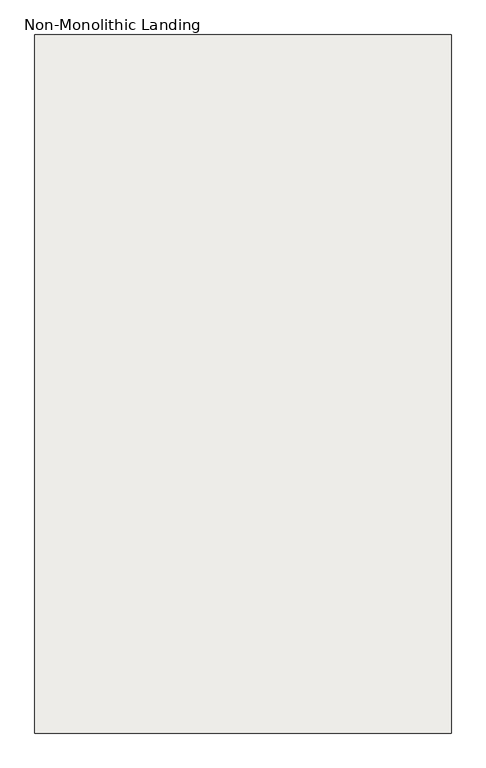
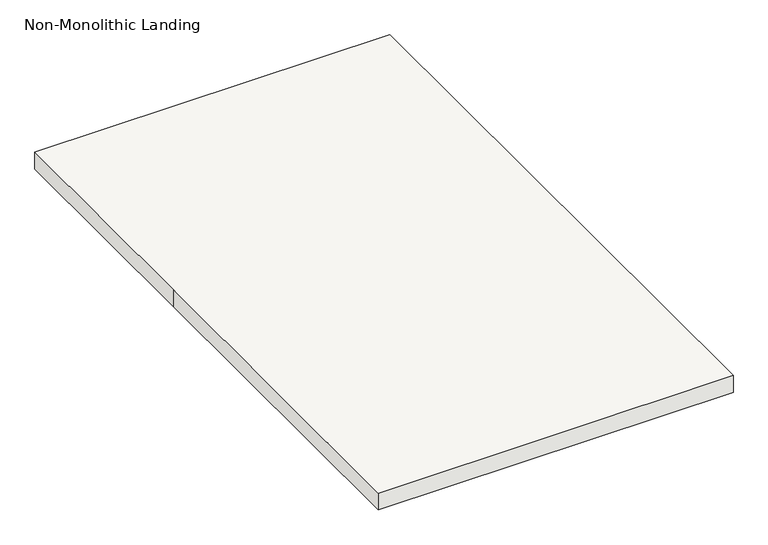
"""IFC4 building model written with IfcOpenShell, lengths in millimetres: slab geometry, Non-Monolithic Landing."""

from ifc_helpers import new_model, si_unit, frame, origin, place, context, project, spatial, polyline, outline, extrude, source, transform, mapped, element, save


def non_monolithic_landing_50201be4(model_context):
    return source(origin(), model_context, "Body", "SweptSolid", [
        extrude(outline(polyline([(21749.836337, -3574.4857187), (21749.836337, -2898.7292651), (22749.836337, -2898.7292651), (22749.836337, -4574.4857187), (21749.836337, -4574.4857187), (21749.836337, -3574.4857187)])), frame((0.0, 0.0, 4630.0), z_axis=(0.0, 0.0, 1.0), x_axis=(1.0, 0.0, 0.0)), (0.0, 0.0, 1.0), 50.0),
    ])


if __name__ == "__main__":
    model = new_model("IFC4")
    model_context = context("Model", 3, world=origin())
    ifc_project = project(units=[si_unit("LENGTHUNIT", "METRE", prefix="MILLI")], contexts=[model_context])
    site = spatial("IfcSite", under=ifc_project)
    building = spatial("IfcBuilding", under=site)
    placement = place(None, origin())
    non_monolithic_landing_shape = non_monolithic_landing_50201be4(model_context)
    element("IfcSlab", 1, ObjectType="Non-Monolithic Landing", at=placement, inside=building, context=model_context, shape_type="MappedRepresentation", body=[
        mapped(non_monolithic_landing_shape, transform((0.0, 0.0, 0.0), x_axis=(1.0, 0.0, 0.0), y_axis=(0.0, 1.0, 0.0), z_axis=(0.0, 0.0, 1.0))),
    ])
    save(model, "model.ifc")
